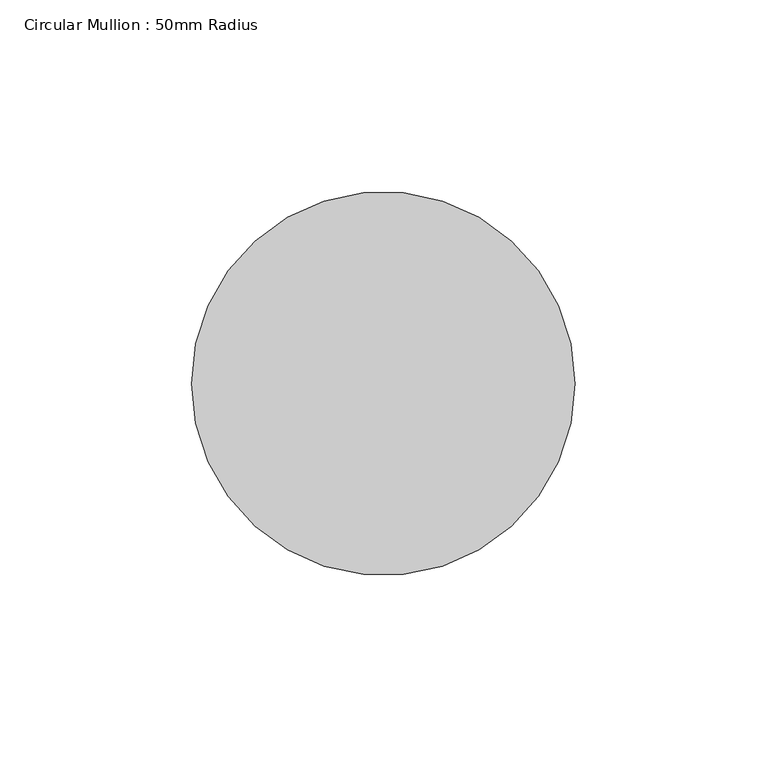
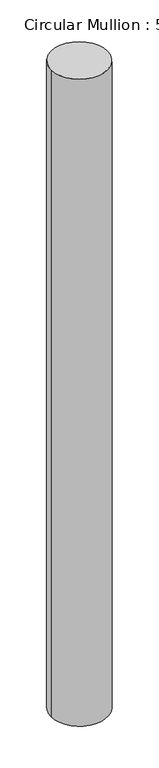
"""IFC4 building model written with IfcOpenShell, lengths in millimetres: member geometry, Circular Mullion : 50mm Radius."""

from ifc_helpers import new_model, si_unit, point, frame, origin, origin_2d, place, context, project, spatial, circle_curve, trimmed, segment, composite_curve, outline, extrude, source, transform, mapped, element, save


def circular_mullion_50mm_radius_13492138(model_context):
    return source(origin(), model_context, "Body", "SweptSolid", [
        extrude(outline(composite_curve([segment(trimmed(circle_curve(origin_2d(), 50.0), [point((50.0, 0.0))], [point((-50.0, 0.0))], False, "CARTESIAN"), True, "CONTINUOUS"), segment(trimmed(circle_curve(origin_2d(), 50.0), [point((-50.0, 0.0))], [point((50.0, 0.0))], False, "CARTESIAN"), True, "CONTINUOUS")], self_intersect=False)), frame((0.0, 0.0, -1209.6912509), z_axis=(0.0, 0.0, 1.0), x_axis=(1.0, 0.0, 0.0)), (0.0, 0.0, 1.0), 1209.6912509),
    ])


if __name__ == "__main__":
    model = new_model("IFC4")
    model_context = context("Model", 3, world=origin())
    ifc_project = project(units=[si_unit("LENGTHUNIT", "METRE", prefix="MILLI")], contexts=[model_context])
    site = spatial("IfcSite", under=ifc_project)
    building = spatial("IfcBuilding", under=site)
    placement = place(None, origin())
    circular_mullion_50mm_radius_shape = circular_mullion_50mm_radius_13492138(model_context)
    element("IfcMember", 1, ObjectType="Circular Mullion : 50mm Radius", at=placement, inside=building, context=model_context, shape_type="MappedRepresentation", body=[
        mapped(circular_mullion_50mm_radius_shape, transform((0.0, 0.0, 0.0), x_axis=(1.0, 0.0, 0.0), y_axis=(0.0, 1.0, 0.0), z_axis=(0.0, 0.0, 1.0))),
    ])
    save(model, "model.ifc")

# Revit data of these elements
# Type "Circular Mullion : 50mm Radius"
#   built-in parameter 1007350 = 0.164042 (stored number, unit not read)
# Element 1 (IfcMember, "Circular Mullion : 50mm Radius")
#   Materials on its faces: "Aluminium"
# Materials
#   "Aluminium": class "Metal", colour RGB 247 247 247, transparency 0, Description = "Aluminium 6061", Cost = 0
